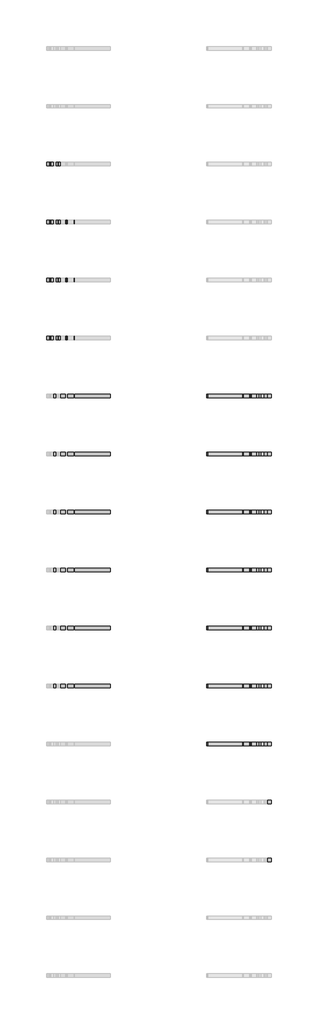
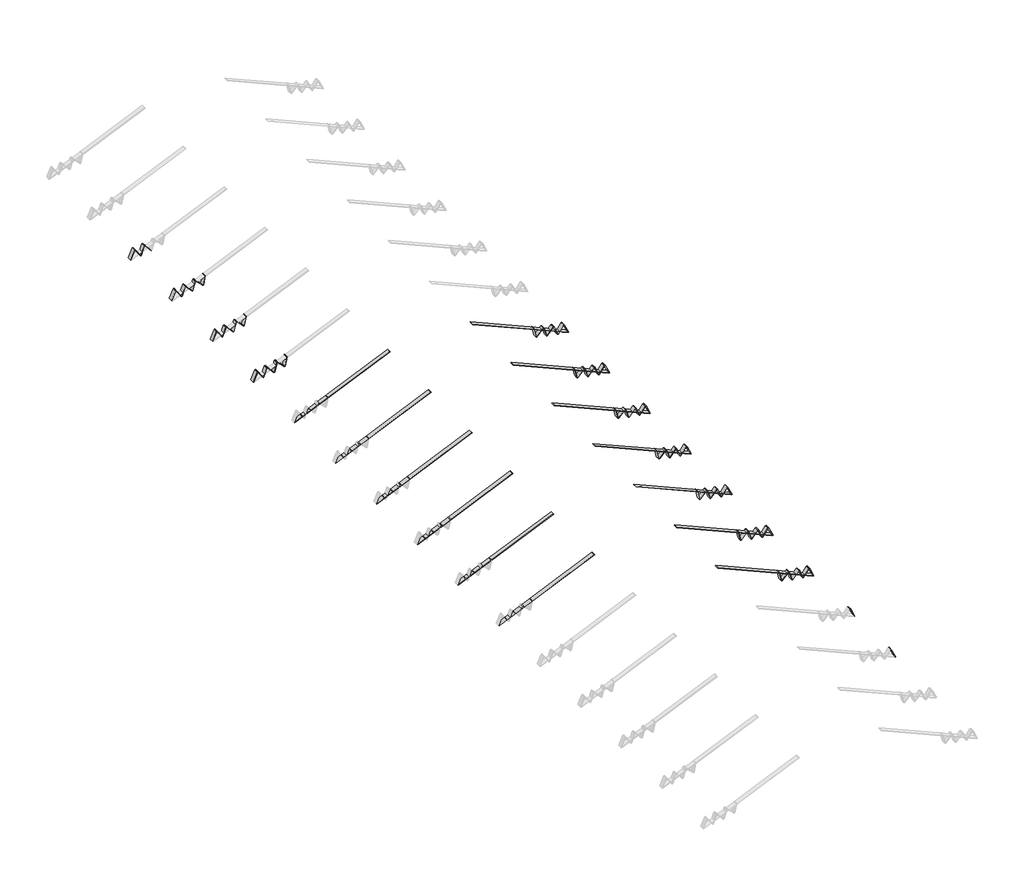
# One storey, part 3 of 4: 89 beams.
"""IFC4 building model written with IfcOpenShell, lengths in millimetres."""

import ifcopenshell
import ifcopenshell.guid

model = None  # the IFC model being written
_history = None  # IfcOwnerHistory: only IFC2X3 demands one
_inside = {}  # id of a spatial element -> (the spatial element, [elements in it])
_under = {}  # id of a project, library or spatial element -> (it, [spatial elements below it])
_declared = {}  # id of a project -> (the project, [libraries it declares])
_typed = {}  # id of a type object -> (the type object, [elements of that type])
_made_of = {}  # id of a material, layer set ... -> (it, [elements and type objects made of it])


def new_model(schema):
    """Start an empty IFC model of exactly this schema.

    Asked for "IFC4X3", IfcOpenShell would pick the latest addendum, in which some entities
    have other attributes; the version numbers below select the first issue.
    IFC2X3 requires an IfcOwnerHistory on every rooted entity: one is made here for all.
    """
    global model, _history
    if schema == "IFC4X3":
        model = ifcopenshell.file(schema_version=(4, 3, 0, 0))
    else:
        model = ifcopenshell.file(schema=schema)
    _inside.clear()
    _under.clear()
    _declared.clear()
    _typed.clear()
    _made_of.clear()
    _history = None
    if model.schema == "IFC2X3":
        org = make("IfcOrganization", Name="unknown")
        user = make(
            "IfcPersonAndOrganization",
            ThePerson=make("IfcPerson", FamilyName="unknown"),
            TheOrganization=org,
        )
        app = make(
            "IfcApplication",
            ApplicationDeveloper=org,
            Version="unknown",
            ApplicationFullName="unknown",
            ApplicationIdentifier="unknown",
        )
        _history = make(
            "IfcOwnerHistory",
            OwningUser=user,
            OwningApplication=app,
            ChangeAction="ADDED",
            CreationDate=0,
        )
    return model


def make(cls, **values):
    """One entity of the class cls with the attributes given. An attribute that is None is left unset."""
    return model.create_entity(
        cls, **{name: value for name, value in values.items() if value is not None}
    )


def rooted(cls, **values):
    """An entity with a GlobalId (a new one), such as an element, a storey or a relation."""
    return make(cls, GlobalId=ifcopenshell.guid.new(), OwnerHistory=_history, **values)


def si_unit(unit_type, name, prefix=None):
    """IfcSIUnit, for example si_unit("LENGTHUNIT", "METRE", prefix="MILLI")."""
    return make("IfcSIUnit", UnitType=unit_type, Prefix=prefix, Name=name)


def assignment(units):
    """IfcUnitAssignment: the units of a project."""
    return None if units is None else make("IfcUnitAssignment", Units=units)


def point(xyz):
    """IfcCartesianPoint."""
    return None if xyz is None else make("IfcCartesianPoint", Coordinates=xyz)


def direction(xyz):
    """IfcDirection."""
    return None if xyz is None else make("IfcDirection", DirectionRatios=xyz)


def frame(location, z_axis=None, x_axis=None):
    """IfcAxis2Placement3D, a coordinate frame: its origin and axes. An axis left out is left unset."""
    return make(
        "IfcAxis2Placement3D",
        Location=point(location),
        Axis=direction(z_axis),
        RefDirection=direction(x_axis),
    )


def frame_2d(location, x_axis=None):
    """IfcAxis2Placement2D, a coordinate frame in the plane: its origin and x axis."""
    return make(
        "IfcAxis2Placement2D", Location=point(location), RefDirection=direction(x_axis)
    )


def origin():
    """The frame at (0, 0, 0) with its axes left unset."""
    return frame((0.0, 0.0, 0.0))


def place(relative_to, where):
    """IfcLocalPlacement: puts the frame where relative to a parent placement (None: the world)."""
    return make(
        "IfcLocalPlacement", PlacementRelTo=relative_to, RelativePlacement=where
    )


def context(
    kind, dimensions, precision=None, world=None, true_north=None, identifier=None
):
    """IfcGeometricRepresentationContext, for example the 3D "Model" context."""
    return make(
        "IfcGeometricRepresentationContext",
        ContextIdentifier=identifier,
        ContextType=kind,
        CoordinateSpaceDimension=dimensions,
        Precision=precision,
        WorldCoordinateSystem=world,
        TrueNorth=true_north,
    )


def project(units=None, contexts=None):
    """IfcProject with its units and contexts."""
    return rooted(
        "IfcProject",
        Name="project",
        RepresentationContexts=contexts,
        UnitsInContext=assignment(units),
    )


def spatial(cls, under=None, at=None, **own):
    """A site, building, storey or space (cls), placed at a placement, below another one or the project."""
    s = rooted(cls, ObjectPlacement=at, **own)
    if under is not None:
        _under.setdefault(under.id(), (under, []))[1].append(s)
    return s


def polyline(points):
    """IfcPolyline through the points."""
    return make("IfcPolyline", Points=[point(p) for p in points])


def circle_curve(where, radius):
    """IfcCircle in the frame where."""
    return make("IfcCircle", Position=where, Radius=radius)


def trimmed(basis, trim1, trim2, sense, master):
    """IfcTrimmedCurve: the piece of a basis curve between two trims."""
    return make(
        "IfcTrimmedCurve",
        BasisCurve=basis,
        Trim1=trim1,
        Trim2=trim2,
        SenseAgreement=sense,
        MasterRepresentation=master,
    )


def segment(curve, same_sense, transition):
    """IfcCompositeCurveSegment."""
    return make(
        "IfcCompositeCurveSegment",
        Transition=transition,
        SameSense=same_sense,
        ParentCurve=curve,
    )


def composite_curve(segments, self_intersect=None):
    """IfcCompositeCurve: segments joined end to end."""
    return make("IfcCompositeCurve", Segments=segments, SelfIntersect=self_intersect)


def outline(outer, holes=None, kind="AREA"):
    """IfcArbitraryClosedProfileDef: a profile drawn as a closed curve; with holes, ...WithVoids."""
    if holes is None:
        return make("IfcArbitraryClosedProfileDef", ProfileType=kind, OuterCurve=outer)
    return make(
        "IfcArbitraryProfileDefWithVoids",
        ProfileType=kind,
        OuterCurve=outer,
        InnerCurves=holes,
    )


def extrude(swept, where, along, depth):
    """IfcExtrudedAreaSolid: the profile swept, set in the frame where, extruded along a direction by depth."""
    return make(
        "IfcExtrudedAreaSolid",
        SweptArea=swept,
        Position=where,
        ExtrudedDirection=direction(along),
        Depth=depth,
    )


def shape(context_of_items, identifier, shape_type, items):
    """IfcShapeRepresentation: the items that make up one representation, for example the "Body"."""
    return make(
        "IfcShapeRepresentation",
        ContextOfItems=context_of_items,
        RepresentationIdentifier=identifier,
        RepresentationType=shape_type,
        Items=items,
    )


def source(mapping_origin, context_of_items, identifier, shape_type, items):
    """IfcRepresentationMap: a shape defined once, which mapped items show again and again."""
    return make(
        "IfcRepresentationMap",
        MappingOrigin=mapping_origin,
        MappedRepresentation=shape(context_of_items, identifier, shape_type, items),
    )


def transform(
    local_origin,
    x_axis=None,
    y_axis=None,
    z_axis=None,
    scale=None,
    scale2=None,
    scale3=None,
    uniform=True,
):
    """IfcCartesianTransformationOperator3D, or its non-uniform kind. x_axis, y_axis, z_axis: its Axis1, 2, 3."""
    if uniform:
        return make(
            "IfcCartesianTransformationOperator3D",
            Axis1=direction(x_axis),
            Axis2=direction(y_axis),
            LocalOrigin=point(local_origin),
            Scale=scale,
            Axis3=direction(z_axis),
        )
    return make(
        "IfcCartesianTransformationOperator3DnonUniform",
        Axis1=direction(x_axis),
        Axis2=direction(y_axis),
        LocalOrigin=point(local_origin),
        Scale=scale,
        Axis3=direction(z_axis),
        Scale2=scale2,
        Scale3=scale3,
    )


def mapped(mapping_source, mapping_target):
    """IfcMappedItem: shows the shape of a source again, moved by a transform."""
    return make(
        "IfcMappedItem", MappingSource=mapping_source, MappingTarget=mapping_target
    )


def made_of(thing, what):
    """Note that an element or type object is made of a material, layer set ...; save() writes the relation."""
    if what is not None:
        _made_of.setdefault(what.id(), (what, []))[1].append(thing)
    return thing


def element(
    cls,
    number,
    at=None,
    inside=None,
    cuts=None,
    type_object=None,
    material=None,
    context=None,
    identifier="Body",
    shape_type=None,
    held_by="IfcProductDefinitionShape",
    body=None,
    shapes=None,
    **own,
):
    """One element of the class cls, such as IfcWall. Its Tag is "e" and its number.

    at: its placement. inside: the storey or other place that contains it. cuts: it is an
    opening in that element (IfcRelVoidsElement). A single representation is given by context,
    identifier, shape_type and body (its items); several are given by shapes. held_by: the class
    of the entity that holds the representations. save() writes the other relations.
    """
    e = rooted(cls, Tag="e%d" % number, ObjectPlacement=at, **own)
    if body is not None:
        shapes = [shape(context, identifier, shape_type, body)]
    if shapes is not None:
        e.Representation = make(held_by, Representations=shapes)
    if inside is not None:
        _inside.setdefault(inside.id(), (inside, []))[1].append(e)
    if cuts is not None:
        rooted(
            "IfcRelVoidsElement", RelatingBuildingElement=cuts, RelatedOpeningElement=e
        )
    if type_object is not None:
        _typed.setdefault(type_object.id(), (type_object, []))[1].append(e)
    return made_of(e, material)


def aggregate(whole, parts):
    """IfcRelAggregates: a whole, such as a stair, and the parts it consists of."""
    return rooted("IfcRelAggregates", RelatingObject=whole, RelatedObjects=parts)


def save(model, path):
    """Write the relations noted so far, then the file.

    IfcRelAggregates (storeys below a building ...), IfcRelContainedInSpatialStructure (elements
    in a storey), IfcRelDefinesByType, IfcRelAssociatesMaterial and IfcRelDeclares: one each for
    every whole, place, type object, material and project.
    """
    for whole, parts in _under.values():
        aggregate(whole, parts)
    for where, things in _inside.values():
        rooted(
            "IfcRelContainedInSpatialStructure",
            RelatedElements=things,
            RelatingStructure=where,
        )
    for kind, things in _typed.values():
        rooted("IfcRelDefinesByType", RelatedObjects=things, RelatingType=kind)
    for what, things in _made_of.values():
        rooted("IfcRelAssociatesMaterial", RelatedObjects=things, RelatingMaterial=what)
    for by, libraries in _declared.values():
        rooted("IfcRelDeclares", RelatingContext=by, RelatedDefinitions=libraries)
    model.write(path)


def placa_diagonal_a71479e9(model_context):
    return source(origin(), model_context, "Body", "SweptSolid", [
        extrude(outline(polyline([(161.178496, 75.0), (161.178496, -75.0), (-185.3041805, -75.0), (-185.3041805, 75.0), (161.178496, 75.0)])), frame((0.0, 0.0, -4.0), z_axis=(0.0, 0.0, 1.0), x_axis=(1.0, 0.0, 0.0)), (0.0, 0.0, 1.0), 8.0),
    ])


def placa_diagonal_67ce8334(model_context):
    return source(origin(), model_context, "Body", "SweptSolid", [
        extrude(outline(polyline([(162.9623469, 75.0), (162.9623469, -75.0), (-162.6761246, -75.0), (-162.6761246, 75.0), (162.9623469, 75.0)])), frame((0.0, 0.0, -4.0), z_axis=(0.0, 0.0, 1.0), x_axis=(1.0, 0.0, 0.0)), (0.0, 0.0, 1.0), 8.0),
    ])


def placa_diagonal_af2a04a3(model_context):
    return source(origin(), model_context, "Body", "SweptSolid", [
        extrude(outline(polyline([(165.1705216, 75.0), (165.1705216, -75.0), (-165.4962729, -75.0), (-165.4962729, 75.0), (165.1705216, 75.0)])), frame((0.0, 0.0, -4.0), z_axis=(0.0, 0.0, 1.0), x_axis=(1.0, 0.0, 0.0)), (0.0, 0.0, 1.0), 8.0),
    ])


def placa_diagonal_fb53ba7d(model_context):
    return source(origin(), model_context, "Body", "SweptSolid", [
        extrude(outline(polyline([(169.971959, 75.0), (169.971959, -75.0), (-169.5739242, -75.0), (-169.5739242, 75.0), (169.971959, 75.0)])), frame((0.0, 0.0, -4.0), z_axis=(0.0, 0.0, 1.0), x_axis=(1.0, 0.0, 0.0)), (0.0, 0.0, 1.0), 8.0),
    ])


def placa_diagonal_d1da0e1c(model_context):
    return source(origin(), model_context, "Body", "SweptSolid", [
        extrude(outline(polyline([(165.1705221, 75.0), (165.1705221, -75.0), (-165.4962734, -75.0), (-165.4962734, 75.0), (165.1705221, 75.0)])), frame((0.0, 0.0, -4.0), z_axis=(0.0, 0.0, 1.0), x_axis=(1.0, 0.0, 0.0)), (0.0, 0.0, 1.0), 8.0),
    ])


def placa_diagonal_6d03bdc5(model_context):
    return source(origin(), model_context, "Body", "SweptSolid", [
        extrude(outline(polyline([(191.209825, 75.0), (191.209825, -75.0), (-166.9394885, -75.0), (-166.9394885, 75.0), (191.209825, 75.0)])), frame((0.0, 0.0, -4.0), z_axis=(0.0, 0.0, 1.0), x_axis=(1.0, 0.0, 0.0)), (0.0, 0.0, 1.0), 8.0),
    ])


def placa_diagonal_30fa4039(model_context):
    return source(origin(), model_context, "Body", "SweptSolid", [
        extrude(outline(polyline([(167.0675386, 75.0), (167.0675386, -75.0), (-167.4240159, -75.0), (-167.4240159, 75.0), (167.0675386, 75.0)])), frame((0.0, 0.0, -4.0), z_axis=(0.0, 0.0, 1.0), x_axis=(1.0, 0.0, 0.0)), (0.0, 0.0, 1.0), 8.0),
    ])


def placa_diagonal_ded414cc(model_context):
    return source(origin(), model_context, "Body", "SweptSolid", [
        extrude(outline(polyline([(167.4240165, 75.0), (167.4240165, -75.0), (-167.0675392, -75.0), (-167.0675392, 75.0), (167.4240165, 75.0)])), frame((0.0, 0.0, -4.0), z_axis=(0.0, 0.0, 1.0), x_axis=(1.0, 0.0, 0.0)), (0.0, 0.0, 1.0), 8.0),
    ])


def placa_diagonal_4690b74a(model_context):
    return source(origin(), model_context, "Body", "SweptSolid", [
        extrude(outline(polyline([(167.0675389, 75.0), (167.0675389, -75.0), (-167.4240162, -75.0), (-167.4240162, 75.0), (167.0675389, 75.0)])), frame((0.0, 0.0, -4.0), z_axis=(0.0, 0.0, 1.0), x_axis=(1.0, 0.0, 0.0)), (0.0, 0.0, 1.0), 8.0),
    ])


def placa_diagonal_aaf0c3b6(model_context):
    return source(origin(), model_context, "Body", "SweptSolid", [
        extrude(outline(polyline([(167.4240163, 75.0), (167.4240163, -75.0), (-167.067539, -75.0), (-167.067539, 75.0), (167.4240163, 75.0)])), frame((0.0, 0.0, -4.0), z_axis=(0.0, 0.0, 1.0), x_axis=(1.0, 0.0, 0.0)), (0.0, 0.0, 1.0), 8.0),
    ])


model = new_model("IFC4")

# Units and contexts
model_context = context("Model", 3, world=origin())
ifc_project = project(units=[si_unit("LENGTHUNIT", "METRE", prefix="MILLI")], contexts=[model_context])

# Site, building, storey
site = spatial("IfcSite", under=ifc_project)
building = spatial("IfcBuilding", under=site)
storey = spatial("IfcBuildingStorey", under=building, Name="Nível 4", Elevation=48165.0)

# Beams
placement = place(None, origin())
element("IfcBeam", 1, ObjectType="Placa : banzo", at=placement, inside=storey, context=model_context, shape_type="SweptSolid", body=[
    extrude(outline(composite_curve([segment(polyline([(48158.5516223, 8114.9704041), (48174.5198715, 8115.9778843)]), True, "CONTINUOUS"), segment(trimmed(circle_curve(frame_2d((53506.1312788, 8452.3636953)), 5342.2126139), [point((48174.5198715, 8115.9778843))], [point((49646.1683419, 4759.1372282))], True, "CARTESIAN"), True, "CONTINUOUS"), segment(polyline([(49646.1683419, 4759.1372282), (49634.6077, 4748.0759643)]), True, "CONTINUOUS"), segment(trimmed(circle_curve(frame_2d((53506.1312788, 8452.3636953)), 5358.2126139), [point((49634.6077, 4748.0759643))], [point((48158.5516223, 8114.9704041))], False, "CARTESIAN"), True, "CONTINUOUS")], self_intersect=False)), frame((0.0, -2178.5623634, 0.0), z_axis=(0.0, 1.0, 0.0), x_axis=(0.0, 0.0, 1.0)), (0.0, 0.0, 1.0), 150.0),
])
element("IfcBeam", 2, ObjectType="Placa : banzo", at=placement, inside=storey, context=model_context, shape_type="SweptSolid", body=[
    extrude(outline(composite_curve([segment(polyline([(49634.6077, 1843.8240278), (49646.1683419, 1832.762764)]), True, "CONTINUOUS"), segment(trimmed(circle_curve(frame_2d((53506.1312788, -1860.4637031)), 5342.2126139), [point((49646.1683419, 1832.762764))], [point((48174.5198715, -1524.0778921))], True, "CARTESIAN"), True, "CONTINUOUS"), segment(polyline([(48174.5198715, -1524.0778921), (48158.5516223, -1523.070412)]), True, "CONTINUOUS"), segment(trimmed(circle_curve(frame_2d((53506.1312788, -1860.4637031)), 5358.2126139), [point((48158.5516223, -1523.070412))], [point((49634.6077, 1843.8240278))], False, "CARTESIAN"), True, "CONTINUOUS")], self_intersect=False)), frame((0.0, -2178.5623634, 0.0), z_axis=(0.0, 1.0, 0.0), x_axis=(0.0, 0.0, 1.0)), (0.0, 0.0, 1.0), 150.0),
])
element("IfcBeam", 3, ObjectType="Placa : banzo", at=placement, inside=storey, context=model_context, shape_type="SweptSolid", body=[
    extrude(outline(composite_curve([segment(polyline([(48158.5516223, 8114.9704041), (48174.5198715, 8115.9778843)]), True, "CONTINUOUS"), segment(trimmed(circle_curve(frame_2d((53506.1312788, 8452.3636953)), 5342.2126139), [point((48174.5198715, 8115.9778843))], [point((49646.1683419, 4759.1372282))], True, "CARTESIAN"), True, "CONTINUOUS"), segment(polyline([(49646.1683419, 4759.1372282), (49634.6077, 4748.0759643)]), True, "CONTINUOUS"), segment(trimmed(circle_curve(frame_2d((53506.1312788, 8452.3636953)), 5358.2126139), [point((49634.6077, 4748.0759643))], [point((48158.5516223, 8114.9704041))], False, "CARTESIAN"), True, "CONTINUOUS")], self_intersect=False)), frame((0.0, -4678.5623634, 0.0), z_axis=(0.0, 1.0, 0.0), x_axis=(0.0, 0.0, 1.0)), (0.0, 0.0, 1.0), 150.0),
])
element("IfcBeam", 4, ObjectType="Placa : banzo", at=placement, inside=storey, context=model_context, shape_type="SweptSolid", body=[
    extrude(outline(composite_curve([segment(polyline([(49634.6077, 1843.8240278), (49646.1683419, 1832.762764)]), True, "CONTINUOUS"), segment(trimmed(circle_curve(frame_2d((53506.1312788, -1860.4637031)), 5342.2126139), [point((49646.1683419, 1832.762764))], [point((48174.5198715, -1524.0778921))], True, "CARTESIAN"), True, "CONTINUOUS"), segment(polyline([(48174.5198715, -1524.0778921), (48158.5516223, -1523.070412)]), True, "CONTINUOUS"), segment(trimmed(circle_curve(frame_2d((53506.1312788, -1860.4637031)), 5358.2126139), [point((48158.5516223, -1523.070412))], [point((49634.6077, 1843.8240278))], False, "CARTESIAN"), True, "CONTINUOUS")], self_intersect=False)), frame((0.0, -4678.5623634, 0.0), z_axis=(0.0, 1.0, 0.0), x_axis=(0.0, 0.0, 1.0)), (0.0, 0.0, 1.0), 150.0),
])
element("IfcBeam", 5, ObjectType="Placa : banzo", at=placement, inside=storey, context=model_context, shape_type="SweptSolid", body=[
    extrude(outline(composite_curve([segment(polyline([(48158.5516223, 8114.9704041), (48174.5198715, 8115.9778843)]), True, "CONTINUOUS"), segment(trimmed(circle_curve(frame_2d((53506.1312788, 8452.3636953)), 5342.2126139), [point((48174.5198715, 8115.9778843))], [point((49646.1683419, 4759.1372282))], True, "CARTESIAN"), True, "CONTINUOUS"), segment(polyline([(49646.1683419, 4759.1372282), (49634.6077, 4748.0759643)]), True, "CONTINUOUS"), segment(trimmed(circle_curve(frame_2d((53506.1312788, 8452.3636953)), 5358.2126139), [point((49634.6077, 4748.0759643))], [point((48158.5516223, 8114.9704041))], False, "CARTESIAN"), True, "CONTINUOUS")], self_intersect=False)), frame((0.0, -7178.5623634, 0.0), z_axis=(0.0, 1.0, 0.0), x_axis=(0.0, 0.0, 1.0)), (0.0, 0.0, 1.0), 150.0),
])
element("IfcBeam", 6, ObjectType="Placa : banzo", at=placement, inside=storey, context=model_context, shape_type="SweptSolid", body=[
    extrude(outline(composite_curve([segment(polyline([(49634.6077, 1843.8240278), (49646.1683419, 1832.762764)]), True, "CONTINUOUS"), segment(trimmed(circle_curve(frame_2d((53506.1312788, -1860.4637031)), 5342.2126139), [point((49646.1683419, 1832.762764))], [point((48174.5198715, -1524.0778921))], True, "CARTESIAN"), True, "CONTINUOUS"), segment(polyline([(48174.5198715, -1524.0778921), (48158.5516223, -1523.070412)]), True, "CONTINUOUS"), segment(trimmed(circle_curve(frame_2d((53506.1312788, -1860.4637031)), 5358.2126139), [point((48158.5516223, -1523.070412))], [point((49634.6077, 1843.8240278))], False, "CARTESIAN"), True, "CONTINUOUS")], self_intersect=False)), frame((0.0, -7178.5623634, 0.0), z_axis=(0.0, 1.0, 0.0), x_axis=(0.0, 0.0, 1.0)), (0.0, 0.0, 1.0), 150.0),
])
element("IfcBeam", 7, ObjectType="Placa : banzo", at=placement, inside=storey, context=model_context, shape_type="SweptSolid", body=[
    extrude(outline(composite_curve([segment(polyline([(48158.5516223, 8114.9704041), (48174.5198715, 8115.9778843)]), True, "CONTINUOUS"), segment(trimmed(circle_curve(frame_2d((53506.1312788, 8452.3636953)), 5342.2126139), [point((48174.5198715, 8115.9778843))], [point((49646.1683419, 4759.1372282))], True, "CARTESIAN"), True, "CONTINUOUS"), segment(polyline([(49646.1683419, 4759.1372282), (49634.6077, 4748.0759643)]), True, "CONTINUOUS"), segment(trimmed(circle_curve(frame_2d((53506.1312788, 8452.3636953)), 5358.2126139), [point((49634.6077, 4748.0759643))], [point((48158.5516223, 8114.9704041))], False, "CARTESIAN"), True, "CONTINUOUS")], self_intersect=False)), frame((0.0, -9678.5623634, 0.0), z_axis=(0.0, 1.0, 0.0), x_axis=(0.0, 0.0, 1.0)), (0.0, 0.0, 1.0), 150.0),
])
element("IfcBeam", 8, ObjectType="Placa : banzo", at=placement, inside=storey, context=model_context, shape_type="SweptSolid", body=[
    extrude(outline(composite_curve([segment(polyline([(49634.6077, 1843.8240278), (49646.1683419, 1832.762764)]), True, "CONTINUOUS"), segment(trimmed(circle_curve(frame_2d((53506.1312788, -1860.4637031)), 5342.2126139), [point((49646.1683419, 1832.762764))], [point((48174.5198715, -1524.0778921))], True, "CARTESIAN"), True, "CONTINUOUS"), segment(polyline([(48174.5198715, -1524.0778921), (48158.5516223, -1523.070412)]), True, "CONTINUOUS"), segment(trimmed(circle_curve(frame_2d((53506.1312788, -1860.4637031)), 5358.2126139), [point((48158.5516223, -1523.070412))], [point((49634.6077, 1843.8240278))], False, "CARTESIAN"), True, "CONTINUOUS")], self_intersect=False)), frame((0.0, -9678.5623634, 0.0), z_axis=(0.0, 1.0, 0.0), x_axis=(0.0, 0.0, 1.0)), (0.0, 0.0, 1.0), 150.0),
])
element("IfcBeam", 9, ObjectType="Placa : banzo", at=placement, inside=storey, context=model_context, shape_type="SweptSolid", body=[
    extrude(outline(composite_curve([segment(polyline([(48158.5516223, 8114.9704041), (48174.5198715, 8115.9778843)]), True, "CONTINUOUS"), segment(trimmed(circle_curve(frame_2d((53506.1312788, 8452.3636953)), 5342.2126139), [point((48174.5198715, 8115.9778843))], [point((49646.1683419, 4759.1372282))], True, "CARTESIAN"), True, "CONTINUOUS"), segment(polyline([(49646.1683419, 4759.1372282), (49634.6077, 4748.0759643)]), True, "CONTINUOUS"), segment(trimmed(circle_curve(frame_2d((53506.1312788, 8452.3636953)), 5358.2126139), [point((49634.6077, 4748.0759643))], [point((48158.5516223, 8114.9704041))], False, "CARTESIAN"), True, "CONTINUOUS")], self_intersect=False)), frame((0.0, -12178.5623634, 0.0), z_axis=(0.0, 1.0, 0.0), x_axis=(0.0, 0.0, 1.0)), (0.0, 0.0, 1.0), 150.0),
])
element("IfcBeam", 10, ObjectType="Placa : banzo", at=placement, inside=storey, context=model_context, shape_type="SweptSolid", body=[
    extrude(outline(composite_curve([segment(polyline([(49634.6077, 1843.8240278), (49646.1683419, 1832.762764)]), True, "CONTINUOUS"), segment(trimmed(circle_curve(frame_2d((53506.1312788, -1860.4637031)), 5342.2126139), [point((49646.1683419, 1832.762764))], [point((48174.5198715, -1524.0778921))], True, "CARTESIAN"), True, "CONTINUOUS"), segment(polyline([(48174.5198715, -1524.0778921), (48158.5516223, -1523.070412)]), True, "CONTINUOUS"), segment(trimmed(circle_curve(frame_2d((53506.1312788, -1860.4637031)), 5358.2126139), [point((48158.5516223, -1523.070412))], [point((49634.6077, 1843.8240278))], False, "CARTESIAN"), True, "CONTINUOUS")], self_intersect=False)), frame((0.0, -12178.5623634, 0.0), z_axis=(0.0, 1.0, 0.0), x_axis=(0.0, 0.0, 1.0)), (0.0, 0.0, 1.0), 150.0),
])
element("IfcBeam", 11, ObjectType="Placa : banzo", at=placement, inside=storey, context=model_context, shape_type="SweptSolid", body=[
    extrude(outline(composite_curve([segment(polyline([(48158.5516223, 8114.9704041), (48174.5198715, 8115.9778843)]), True, "CONTINUOUS"), segment(trimmed(circle_curve(frame_2d((53506.1312788, 8452.3636953)), 5342.2126139), [point((48174.5198715, 8115.9778843))], [point((49646.1683419, 4759.1372282))], True, "CARTESIAN"), True, "CONTINUOUS"), segment(polyline([(49646.1683419, 4759.1372282), (49634.6077, 4748.0759643)]), True, "CONTINUOUS"), segment(trimmed(circle_curve(frame_2d((53506.1312788, 8452.3636953)), 5358.2126139), [point((49634.6077, 4748.0759643))], [point((48158.5516223, 8114.9704041))], False, "CARTESIAN"), True, "CONTINUOUS")], self_intersect=False)), frame((0.0, -14678.5623634, 0.0), z_axis=(0.0, 1.0, 0.0), x_axis=(0.0, 0.0, 1.0)), (0.0, 0.0, 1.0), 150.0),
])
element("IfcBeam", 12, ObjectType="Placa : banzo", at=placement, inside=storey, context=model_context, shape_type="SweptSolid", body=[
    extrude(outline(composite_curve([segment(polyline([(49634.6077, 1843.8240278), (49646.1683419, 1832.762764)]), True, "CONTINUOUS"), segment(trimmed(circle_curve(frame_2d((53506.1312788, -1860.4637031)), 5342.2126139), [point((49646.1683419, 1832.762764))], [point((48174.5198715, -1524.0778921))], True, "CARTESIAN"), True, "CONTINUOUS"), segment(polyline([(48174.5198715, -1524.0778921), (48158.5516223, -1523.070412)]), True, "CONTINUOUS"), segment(trimmed(circle_curve(frame_2d((53506.1312788, -1860.4637031)), 5358.2126139), [point((48158.5516223, -1523.070412))], [point((49634.6077, 1843.8240278))], False, "CARTESIAN"), True, "CONTINUOUS")], self_intersect=False)), frame((0.0, -14678.5623634, 0.0), z_axis=(0.0, 1.0, 0.0), x_axis=(0.0, 0.0, 1.0)), (0.0, 0.0, 1.0), 150.0),
])
element("IfcBeam", 13, ObjectType="Placa : banzo", at=placement, inside=storey, context=model_context, shape_type="SweptSolid", body=[
    extrude(outline(composite_curve([segment(polyline([(48158.5516223, 8114.9704041), (48174.5198715, 8115.9778843)]), True, "CONTINUOUS"), segment(trimmed(circle_curve(frame_2d((53506.1312788, 8452.3636953)), 5342.2126139), [point((48174.5198715, 8115.9778843))], [point((49646.1683419, 4759.1372282))], True, "CARTESIAN"), True, "CONTINUOUS"), segment(polyline([(49646.1683419, 4759.1372282), (49634.6077, 4748.0759643)]), True, "CONTINUOUS"), segment(trimmed(circle_curve(frame_2d((53506.1312788, 8452.3636953)), 5358.2126139), [point((49634.6077, 4748.0759643))], [point((48158.5516223, 8114.9704041))], False, "CARTESIAN"), True, "CONTINUOUS")], self_intersect=False)), frame((0.0, -17178.5623634, 0.0), z_axis=(0.0, 1.0, 0.0), x_axis=(0.0, 0.0, 1.0)), (0.0, 0.0, 1.0), 150.0),
])
placa_diagonal_shape = placa_diagonal_a71479e9(model_context)
element("IfcBeam", 14, ObjectType="Placa : diagonal", at=placement, inside=storey, context=model_context, shape_type="MappedRepresentation", body=[
    mapped(placa_diagonal_shape, transform((-1468.5029422, 7896.4376366, 48342.5238752), x_axis=(0.4074605623535313, 0.0, 0.9132228042085588), y_axis=(0.0, -1.0, 0.0), z_axis=(0.9132228042085588, 0.0, -0.4074605623535313))),
])
element("IfcBeam", 15, ObjectType="Placa : diagonal", at=placement, inside=storey, context=model_context, shape_type="MappedRepresentation", body=[
    mapped(placa_diagonal_shape, transform((-1468.5029422, 5396.4376366, 48342.5238752), x_axis=(0.4074605623535313, 0.0, 0.9132228042085588), y_axis=(0.0, -1.0, 0.0), z_axis=(0.9132228042085588, 0.0, -0.4074605623535313))),
])
element("IfcBeam", 16, ObjectType="Placa : diagonal", at=placement, inside=storey, context=model_context, shape_type="MappedRepresentation", body=[
    mapped(placa_diagonal_shape, transform((-1468.5029422, 2896.4376366, 48342.5238752), x_axis=(0.4074605623535313, 0.0, 0.9132228042085588), y_axis=(0.0, -1.0, 0.0), z_axis=(0.9132228042085588, 0.0, -0.4074605623535313))),
])
element("IfcBeam", 17, ObjectType="Placa : diagonal", at=placement, inside=storey, context=model_context, shape_type="MappedRepresentation", body=[
    mapped(placa_diagonal_shape, transform((-1468.5029422, 396.4376366, 48342.5238752), x_axis=(0.4074605623535313, 0.0, 0.9132228042085588), y_axis=(0.0, -1.0, 0.0), z_axis=(0.9132228042085588, 0.0, -0.4074605623535313))),
])
placa_diagonal_2_shape = placa_diagonal_67ce8334(model_context)
element("IfcBeam", 18, ObjectType="Placa : diagonal", at=placement, inside=storey, context=model_context, shape_type="MappedRepresentation", body=[
    mapped(placa_diagonal_2_shape, transform((-1292.3410904, 7896.4376366, 48354.815057), x_axis=(0.5398932132172984, 0.0, -0.8417335197803998), y_axis=(0.0, -1.0, 0.0), z_axis=(-0.8417335197803998, 0.0, -0.5398932132172984))),
])
element("IfcBeam", 19, ObjectType="Placa : diagonal", at=placement, inside=storey, context=model_context, shape_type="MappedRepresentation", body=[
    mapped(placa_diagonal_2_shape, transform((-1292.3410904, 5396.4376366, 48354.815057), x_axis=(0.5398932132172984, 0.0, -0.8417335197803998), y_axis=(0.0, -1.0, 0.0), z_axis=(-0.8417335197803998, 0.0, -0.5398932132172984))),
])
element("IfcBeam", 20, ObjectType="Placa : diagonal", at=placement, inside=storey, context=model_context, shape_type="MappedRepresentation", body=[
    mapped(placa_diagonal_2_shape, transform((-1292.3410904, 2896.4376366, 48354.815057), x_axis=(0.5398932132172984, 0.0, -0.8417335197803998), y_axis=(0.0, -1.0, 0.0), z_axis=(-0.8417335197803998, 0.0, -0.5398932132172984))),
])
element("IfcBeam", 21, ObjectType="Placa : diagonal", at=placement, inside=storey, context=model_context, shape_type="MappedRepresentation", body=[
    mapped(placa_diagonal_2_shape, transform((-1292.3410904, 396.4376366, 48354.815057), x_axis=(0.5398932132172984, 0.0, -0.8417335197803998), y_axis=(0.0, -1.0, 0.0), z_axis=(-0.8417335197803998, 0.0, -0.5398932132172984))),
])
placa_diagonal_3_shape = placa_diagonal_af2a04a3(model_context)
element("IfcBeam", 22, ObjectType="Placa : diagonal", at=placement, inside=storey, context=model_context, shape_type="MappedRepresentation", body=[
    mapped(placa_diagonal_3_shape, transform((-1127.2550828, 7896.4376366, 48375.8118772), x_axis=(0.3404667803509138, 0.0, 0.940256545564817), y_axis=(0.0, -1.0, 0.0), z_axis=(0.940256545564817, 0.0, -0.3404667803509138))),
])
element("IfcBeam", 23, ObjectType="Placa : diagonal", at=placement, inside=storey, context=model_context, shape_type="MappedRepresentation", body=[
    mapped(placa_diagonal_3_shape, transform((-1127.2550828, 5396.4376366, 48375.8118772), x_axis=(0.3404667803509138, 0.0, 0.940256545564817), y_axis=(0.0, -1.0, 0.0), z_axis=(0.940256545564817, 0.0, -0.3404667803509138))),
])
element("IfcBeam", 24, ObjectType="Placa : diagonal", at=placement, inside=storey, context=model_context, shape_type="MappedRepresentation", body=[
    mapped(placa_diagonal_3_shape, transform((-392.7303205, 5396.4376366, 48535.8666224), x_axis=(0.20085127706480188, 0.0, 0.9796217456250337), y_axis=(0.0, -1.0, 0.0), z_axis=(0.9796217456250337, 0.0, -0.20085127706480188))),
])
element("IfcBeam", 25, ObjectType="Placa : diagonal", at=placement, inside=storey, context=model_context, shape_type="MappedRepresentation", body=[
    mapped(placa_diagonal_3_shape, transform((-1127.2550828, 2896.4376366, 48375.8118772), x_axis=(0.3404667803509138, 0.0, 0.940256545564817), y_axis=(0.0, -1.0, 0.0), z_axis=(0.940256545564817, 0.0, -0.3404667803509138))),
])
element("IfcBeam", 26, ObjectType="Placa : diagonal", at=placement, inside=storey, context=model_context, shape_type="MappedRepresentation", body=[
    mapped(placa_diagonal_3_shape, transform((-392.7303205, 2896.4376366, 48535.8666224), x_axis=(0.20085127706480188, 0.0, 0.9796217456250337), y_axis=(0.0, -1.0, 0.0), z_axis=(0.9796217456250337, 0.0, -0.20085127706480188))),
])
element("IfcBeam", 27, ObjectType="Placa : diagonal", at=placement, inside=storey, context=model_context, shape_type="MappedRepresentation", body=[
    mapped(placa_diagonal_3_shape, transform((-1127.2550828, 396.4376366, 48375.8118772), x_axis=(0.3404667803509138, 0.0, 0.940256545564817), y_axis=(0.0, -1.0, 0.0), z_axis=(0.940256545564817, 0.0, -0.3404667803509138))),
])
element("IfcBeam", 28, ObjectType="Placa : diagonal", at=placement, inside=storey, context=model_context, shape_type="MappedRepresentation", body=[
    mapped(placa_diagonal_3_shape, transform((-392.7303205, 396.4376366, 48535.8666224), x_axis=(0.20085127706480188, 0.0, 0.9796217456250337), y_axis=(0.0, -1.0, 0.0), z_axis=(0.9796217456250337, 0.0, -0.20085127706480188))),
])
placa_diagonal_4_shape = placa_diagonal_fb53ba7d(model_context)
element("IfcBeam", 29, ObjectType="Placa : diagonal", at=placement, inside=storey, context=model_context, shape_type="MappedRepresentation", body=[
    mapped(placa_diagonal_4_shape, transform((-935.6334765, 7896.4376366, 48407.0552778), x_axis=(0.6551223780870831, 0.0, -0.7555227790937377), y_axis=(0.0, -1.0, 0.0), z_axis=(-0.7555227790937377, 0.0, -0.6551223780870831))),
])
element("IfcBeam", 30, ObjectType="Placa : diagonal", at=placement, inside=storey, context=model_context, shape_type="MappedRepresentation", body=[
    mapped(placa_diagonal_4_shape, transform((-935.6334765, 5396.4376366, 48407.0552778), x_axis=(0.6551223780870831, 0.0, -0.7555227790937377), y_axis=(0.0, -1.0, 0.0), z_axis=(-0.7555227790937377, 0.0, -0.6551223780870831))),
])
element("IfcBeam", 31, ObjectType="Placa : diagonal", at=placement, inside=storey, context=model_context, shape_type="MappedRepresentation", body=[
    mapped(placa_diagonal_4_shape, transform((-568.2358431, 5396.4376366, 48487.5623421), x_axis=(0.7081946416059488, 0.0, -0.706017244549042), y_axis=(0.0, -1.0, 0.0), z_axis=(-0.706017244549042, 0.0, -0.7081946416059488))),
])
element("IfcBeam", 32, ObjectType="Placa : diagonal", at=placement, inside=storey, context=model_context, shape_type="MappedRepresentation", body=[
    mapped(placa_diagonal_4_shape, transform((-935.6334765, 2896.4376366, 48407.0552778), x_axis=(0.6551223780870831, 0.0, -0.7555227790937377), y_axis=(0.0, -1.0, 0.0), z_axis=(-0.7555227790937377, 0.0, -0.6551223780870831))),
])
element("IfcBeam", 33, ObjectType="Placa : diagonal", at=placement, inside=storey, context=model_context, shape_type="MappedRepresentation", body=[
    mapped(placa_diagonal_4_shape, transform((-568.2358431, 2896.4376366, 48487.5623421), x_axis=(0.7081946416059488, 0.0, -0.706017244549042), y_axis=(0.0, -1.0, 0.0), z_axis=(-0.706017244549042, 0.0, -0.7081946416059488))),
])
element("IfcBeam", 34, ObjectType="Placa : diagonal", at=placement, inside=storey, context=model_context, shape_type="MappedRepresentation", body=[
    mapped(placa_diagonal_4_shape, transform((-935.6334765, 396.4376366, 48407.0552778), x_axis=(0.6551223780870831, 0.0, -0.7555227790937377), y_axis=(0.0, -1.0, 0.0), z_axis=(-0.7555227790937377, 0.0, -0.6551223780870831))),
])
element("IfcBeam", 35, ObjectType="Placa : diagonal", at=placement, inside=storey, context=model_context, shape_type="MappedRepresentation", body=[
    mapped(placa_diagonal_4_shape, transform((-568.2358431, 396.4376366, 48487.5623421), x_axis=(0.7081946416059488, 0.0, -0.706017244549042), y_axis=(0.0, -1.0, 0.0), z_axis=(-0.706017244549042, 0.0, -0.7081946416059488))),
])
placa_diagonal_5_shape = placa_diagonal_d1da0e1c(model_context)
element("IfcBeam", 36, ObjectType="Placa : diagonal", at=placement, inside=storey, context=model_context, shape_type="MappedRepresentation", body=[
    mapped(placa_diagonal_5_shape, transform((-757.0867023, 5396.4376366, 48442.5030113), x_axis=(0.2713737594345945, 0.0, 0.9624740426059993), y_axis=(0.0, -1.0, 0.0), z_axis=(0.9624740426059993, 0.0, -0.2713737594345945))),
])
element("IfcBeam", 37, ObjectType="Placa : diagonal", at=placement, inside=storey, context=model_context, shape_type="MappedRepresentation", body=[
    mapped(placa_diagonal_5_shape, transform((-757.0867023, 2896.4376366, 48442.5030113), x_axis=(0.2713737594345945, 0.0, 0.9624740426059993), y_axis=(0.0, -1.0, 0.0), z_axis=(0.9624740426059993, 0.0, -0.2713737594345945))),
])
element("IfcBeam", 38, ObjectType="Placa : diagonal", at=placement, inside=storey, context=model_context, shape_type="MappedRepresentation", body=[
    mapped(placa_diagonal_5_shape, transform((-757.0867023, 396.4376366, 48442.5030113), x_axis=(0.2713737594345945, 0.0, 0.9624740426059993), y_axis=(0.0, -1.0, 0.0), z_axis=(0.9624740426059993, 0.0, -0.2713737594345945))),
])
placa_diagonal_6_shape = placa_diagonal_6d03bdc5(model_context)
element("IfcBeam", 39, ObjectType="Placa : diagonal", at=placement, inside=storey, context=model_context, shape_type="MappedRepresentation", body=[
    mapped(placa_diagonal_6_shape, transform((8059.7198757, -2103.5623634, 48338.6280973), x_axis=(0.4189773842608123, 0.0, -0.9079966693099526), y_axis=(0.0, -1.0, 0.0), z_axis=(-0.9079966693099526, 0.0, -0.4189773842608123))),
])
element("IfcBeam", 40, ObjectType="Placa : diagonal", at=placement, inside=storey, context=model_context, shape_type="MappedRepresentation", body=[
    mapped(placa_diagonal_6_shape, transform((8059.7198757, -4603.5623634, 48338.6280973), x_axis=(0.4189773842608123, 0.0, -0.9079966693099526), y_axis=(0.0, -1.0, 0.0), z_axis=(-0.9079966693099526, 0.0, -0.4189773842608123))),
])
element("IfcBeam", 41, ObjectType="Placa : diagonal", at=placement, inside=storey, context=model_context, shape_type="MappedRepresentation", body=[
    mapped(placa_diagonal_6_shape, transform((8059.7198757, -7103.5623634, 48338.6280973), x_axis=(0.4189773842608123, 0.0, -0.9079966693099526), y_axis=(0.0, -1.0, 0.0), z_axis=(-0.9079966693099526, 0.0, -0.4189773842608123))),
])
element("IfcBeam", 42, ObjectType="Placa : diagonal", at=placement, inside=storey, context=model_context, shape_type="MappedRepresentation", body=[
    mapped(placa_diagonal_6_shape, transform((8059.7198757, -9603.5623634, 48338.6280973), x_axis=(0.4189773842608123, 0.0, -0.9079966693099526), y_axis=(0.0, -1.0, 0.0), z_axis=(-0.9079966693099526, 0.0, -0.4189773842608123))),
])
element("IfcBeam", 43, ObjectType="Placa : diagonal", at=placement, inside=storey, context=model_context, shape_type="MappedRepresentation", body=[
    mapped(placa_diagonal_6_shape, transform((8059.7198757, -12103.5623634, 48338.6280973), x_axis=(0.4189773842608123, 0.0, -0.9079966693099526), y_axis=(0.0, -1.0, 0.0), z_axis=(-0.9079966693099526, 0.0, -0.4189773842608123))),
])
element("IfcBeam", 44, ObjectType="Placa : diagonal", at=placement, inside=storey, context=model_context, shape_type="MappedRepresentation", body=[
    mapped(placa_diagonal_6_shape, transform((8059.7198757, -14603.5623634, 48338.6280973), x_axis=(0.4189773842608123, 0.0, -0.9079966693099526), y_axis=(0.0, -1.0, 0.0), z_axis=(-0.9079966693099526, 0.0, -0.4189773842608123))),
])
element("IfcBeam", 45, ObjectType="Placa : diagonal", at=placement, inside=storey, context=model_context, shape_type="MappedRepresentation", body=[
    mapped(placa_diagonal_6_shape, transform((8059.7198757, -17103.5623634, 48338.6280973), x_axis=(0.4189773842608123, 0.0, -0.9079966693099526), y_axis=(0.0, -1.0, 0.0), z_axis=(-0.9079966693099526, 0.0, -0.4189773842608123))),
])
element("IfcBeam", 46, ObjectType="Placa : diagonal", at=placement, inside=storey, context=model_context, shape_type="MappedRepresentation", body=[
    mapped(placa_diagonal_6_shape, transform((8059.7198757, -19603.5623634, 48338.6280973), x_axis=(0.4189773842608123, 0.0, -0.9079966693099526), y_axis=(0.0, -1.0, 0.0), z_axis=(-0.9079966693099526, 0.0, -0.4189773842608123))),
])
element("IfcBeam", 47, ObjectType="Placa : diagonal", at=placement, inside=storey, context=model_context, shape_type="MappedRepresentation", body=[
    mapped(placa_diagonal_6_shape, transform((8059.7198757, -22103.5623634, 48338.6280973), x_axis=(0.4189773842608123, 0.0, -0.9079966693099526), y_axis=(0.0, -1.0, 0.0), z_axis=(-0.9079966693099526, 0.0, -0.4189773842608123))),
])
placa_diagonal_7_shape = placa_diagonal_30fa4039(model_context)
element("IfcBeam", 48, ObjectType="Placa : diagonal", at=placement, inside=storey, context=model_context, shape_type="MappedRepresentation", body=[
    mapped(placa_diagonal_7_shape, transform((7867.9931921, -2103.5623634, 48356.8132581), x_axis=(0.5832804616623758, 0.0, 0.8122708310920229), y_axis=(0.0, -1.0, 0.0), z_axis=(0.8122708310920229, 0.0, -0.5832804616623758))),
])
element("IfcBeam", 49, ObjectType="Placa : diagonal", at=placement, inside=storey, context=model_context, shape_type="MappedRepresentation", body=[
    mapped(placa_diagonal_7_shape, transform((7867.9931921, -4603.5623634, 48356.8132581), x_axis=(0.5832804616623758, 0.0, 0.8122708310920229), y_axis=(0.0, -1.0, 0.0), z_axis=(0.8122708310920229, 0.0, -0.5832804616623758))),
])
element("IfcBeam", 50, ObjectType="Placa : diagonal", at=placement, inside=storey, context=model_context, shape_type="MappedRepresentation", body=[
    mapped(placa_diagonal_7_shape, transform((7867.9931921, -7103.5623634, 48356.8132581), x_axis=(0.5832804616623758, 0.0, 0.8122708310920229), y_axis=(0.0, -1.0, 0.0), z_axis=(0.8122708310920229, 0.0, -0.5832804616623758))),
])
element("IfcBeam", 51, ObjectType="Placa : diagonal", at=placement, inside=storey, context=model_context, shape_type="MappedRepresentation", body=[
    mapped(placa_diagonal_7_shape, transform((7867.9931921, -9603.5623634, 48356.8132581), x_axis=(0.5832804616623758, 0.0, 0.8122708310920229), y_axis=(0.0, -1.0, 0.0), z_axis=(0.8122708310920229, 0.0, -0.5832804616623758))),
])
element("IfcBeam", 52, ObjectType="Placa : diagonal", at=placement, inside=storey, context=model_context, shape_type="MappedRepresentation", body=[
    mapped(placa_diagonal_7_shape, transform((7867.9931921, -12103.5623634, 48356.8132581), x_axis=(0.5832804616623758, 0.0, 0.8122708310920229), y_axis=(0.0, -1.0, 0.0), z_axis=(0.8122708310920229, 0.0, -0.5832804616623758))),
])
element("IfcBeam", 53, ObjectType="Placa : diagonal", at=placement, inside=storey, context=model_context, shape_type="MappedRepresentation", body=[
    mapped(placa_diagonal_7_shape, transform((7867.9931921, -14603.5623634, 48356.8132581), x_axis=(0.5832804616623758, 0.0, 0.8122708310920229), y_axis=(0.0, -1.0, 0.0), z_axis=(0.8122708310920229, 0.0, -0.5832804616623758))),
])
element("IfcBeam", 54, ObjectType="Placa : diagonal", at=placement, inside=storey, context=model_context, shape_type="MappedRepresentation", body=[
    mapped(placa_diagonal_7_shape, transform((7867.9931921, -17103.5623634, 48356.8132581), x_axis=(0.5832804616623758, 0.0, 0.8122708310920229), y_axis=(0.0, -1.0, 0.0), z_axis=(0.8122708310920229, 0.0, -0.5832804616623758))),
])
placa_diagonal_8_shape = placa_diagonal_ded414cc(model_context)
element("IfcBeam", 55, ObjectType="Placa : diagonal", at=placement, inside=storey, context=model_context, shape_type="MappedRepresentation", body=[
    mapped(placa_diagonal_8_shape, transform((7688.6379629, -2103.5623634, 48380.344708), x_axis=(0.3540062158971715, 0.0, -0.935243069531213), y_axis=(0.0, -1.0, 0.0), z_axis=(-0.935243069531213, 0.0, -0.3540062158971715))),
])
element("IfcBeam", 56, ObjectType="Placa : diagonal", at=placement, inside=storey, context=model_context, shape_type="MappedRepresentation", body=[
    mapped(placa_diagonal_8_shape, transform((7321.1773395, -2103.5623634, 48448.7226144), x_axis=(0.2856767726847757, 0.0, -0.9583260309249723), y_axis=(0.0, -1.0, 0.0), z_axis=(-0.9583260309249723, 0.0, -0.2856767726847757))),
])
element("IfcBeam", 57, ObjectType="Placa : diagonal", at=placement, inside=storey, context=model_context, shape_type="MappedRepresentation", body=[
    mapped(placa_diagonal_8_shape, transform((7688.6379629, -4603.5623634, 48380.344708), x_axis=(0.3540062158971715, 0.0, -0.935243069531213), y_axis=(0.0, -1.0, 0.0), z_axis=(-0.935243069531213, 0.0, -0.3540062158971715))),
])
element("IfcBeam", 58, ObjectType="Placa : diagonal", at=placement, inside=storey, context=model_context, shape_type="MappedRepresentation", body=[
    mapped(placa_diagonal_8_shape, transform((7321.1773395, -4603.5623634, 48448.7226144), x_axis=(0.2856767726847757, 0.0, -0.9583260309249723), y_axis=(0.0, -1.0, 0.0), z_axis=(-0.9583260309249723, 0.0, -0.2856767726847757))),
])
element("IfcBeam", 59, ObjectType="Placa : diagonal", at=placement, inside=storey, context=model_context, shape_type="MappedRepresentation", body=[
    mapped(placa_diagonal_8_shape, transform((7688.6379629, -7103.5623634, 48380.344708), x_axis=(0.3540062158971715, 0.0, -0.935243069531213), y_axis=(0.0, -1.0, 0.0), z_axis=(-0.935243069531213, 0.0, -0.3540062158971715))),
])
element("IfcBeam", 60, ObjectType="Placa : diagonal", at=placement, inside=storey, context=model_context, shape_type="MappedRepresentation", body=[
    mapped(placa_diagonal_8_shape, transform((7321.1773395, -7103.5623634, 48448.7226144), x_axis=(0.2856767726847757, 0.0, -0.9583260309249723), y_axis=(0.0, -1.0, 0.0), z_axis=(-0.9583260309249723, 0.0, -0.2856767726847757))),
])
element("IfcBeam", 61, ObjectType="Placa : diagonal", at=placement, inside=storey, context=model_context, shape_type="MappedRepresentation", body=[
    mapped(placa_diagonal_8_shape, transform((7688.6379629, -9603.5623634, 48380.344708), x_axis=(0.3540062158971715, 0.0, -0.935243069531213), y_axis=(0.0, -1.0, 0.0), z_axis=(-0.935243069531213, 0.0, -0.3540062158971715))),
])
element("IfcBeam", 62, ObjectType="Placa : diagonal", at=placement, inside=storey, context=model_context, shape_type="MappedRepresentation", body=[
    mapped(placa_diagonal_8_shape, transform((7321.1773395, -9603.5623634, 48448.7226144), x_axis=(0.2856767726847757, 0.0, -0.9583260309249723), y_axis=(0.0, -1.0, 0.0), z_axis=(-0.9583260309249723, 0.0, -0.2856767726847757))),
])
element("IfcBeam", 63, ObjectType="Placa : diagonal", at=placement, inside=storey, context=model_context, shape_type="MappedRepresentation", body=[
    mapped(placa_diagonal_8_shape, transform((7688.6379629, -12103.5623634, 48380.344708), x_axis=(0.3540062158971715, 0.0, -0.935243069531213), y_axis=(0.0, -1.0, 0.0), z_axis=(-0.935243069531213, 0.0, -0.3540062158971715))),
])
element("IfcBeam", 64, ObjectType="Placa : diagonal", at=placement, inside=storey, context=model_context, shape_type="MappedRepresentation", body=[
    mapped(placa_diagonal_8_shape, transform((7321.1773395, -12103.5623634, 48448.7226144), x_axis=(0.2856767726847757, 0.0, -0.9583260309249723), y_axis=(0.0, -1.0, 0.0), z_axis=(-0.9583260309249723, 0.0, -0.2856767726847757))),
])
element("IfcBeam", 65, ObjectType="Placa : diagonal", at=placement, inside=storey, context=model_context, shape_type="MappedRepresentation", body=[
    mapped(placa_diagonal_8_shape, transform((7688.6379629, -14603.5623634, 48380.344708), x_axis=(0.3540062158971715, 0.0, -0.935243069531213), y_axis=(0.0, -1.0, 0.0), z_axis=(-0.935243069531213, 0.0, -0.3540062158971715))),
])
element("IfcBeam", 66, ObjectType="Placa : diagonal", at=placement, inside=storey, context=model_context, shape_type="MappedRepresentation", body=[
    mapped(placa_diagonal_8_shape, transform((7321.1773395, -14603.5623634, 48448.7226144), x_axis=(0.2856767726847757, 0.0, -0.9583260309249723), y_axis=(0.0, -1.0, 0.0), z_axis=(-0.9583260309249723, 0.0, -0.2856767726847757))),
])
element("IfcBeam", 67, ObjectType="Placa : diagonal", at=placement, inside=storey, context=model_context, shape_type="MappedRepresentation", body=[
    mapped(placa_diagonal_8_shape, transform((7688.6379629, -17103.5623634, 48380.344708), x_axis=(0.3540062158971715, 0.0, -0.935243069531213), y_axis=(0.0, -1.0, 0.0), z_axis=(-0.935243069531213, 0.0, -0.3540062158971715))),
])
element("IfcBeam", 68, ObjectType="Placa : diagonal", at=placement, inside=storey, context=model_context, shape_type="MappedRepresentation", body=[
    mapped(placa_diagonal_8_shape, transform((7321.1773395, -17103.5623634, 48448.7226144), x_axis=(0.2856767726847757, 0.0, -0.9583260309249723), y_axis=(0.0, -1.0, 0.0), z_axis=(-0.9583260309249723, 0.0, -0.2856767726847757))),
])
placa_diagonal_9_shape = placa_diagonal_4690b74a(model_context)
element("IfcBeam", 69, ObjectType="Placa : diagonal", at=placement, inside=storey, context=model_context, shape_type="MappedRepresentation", body=[
    mapped(placa_diagonal_9_shape, transform((7498.370034, -2103.5623634, 48412.3251322), x_axis=(0.6403087836754673, 0.0, 0.7681176091901837), y_axis=(0.0, -1.0, 0.0), z_axis=(0.7681176091901837, 0.0, -0.6403087836754673))),
])
element("IfcBeam", 70, ObjectType="Placa : diagonal", at=placement, inside=storey, context=model_context, shape_type="MappedRepresentation", body=[
    mapped(placa_diagonal_9_shape, transform((7133.7092978, -2103.5623634, 48494.333642), x_axis=(0.6940063880716316, 0.0, 0.719968841906209), y_axis=(0.0, -1.0, 0.0), z_axis=(0.719968841906209, 0.0, -0.6940063880716316))),
])
element("IfcBeam", 71, ObjectType="Placa : diagonal", at=placement, inside=storey, context=model_context, shape_type="MappedRepresentation", body=[
    mapped(placa_diagonal_9_shape, transform((7498.370034, -4603.5623634, 48412.3251322), x_axis=(0.6403087836754673, 0.0, 0.7681176091901837), y_axis=(0.0, -1.0, 0.0), z_axis=(0.7681176091901837, 0.0, -0.6403087836754673))),
])
element("IfcBeam", 72, ObjectType="Placa : diagonal", at=placement, inside=storey, context=model_context, shape_type="MappedRepresentation", body=[
    mapped(placa_diagonal_9_shape, transform((7133.7092978, -4603.5623634, 48494.333642), x_axis=(0.6940063880716316, 0.0, 0.719968841906209), y_axis=(0.0, -1.0, 0.0), z_axis=(0.719968841906209, 0.0, -0.6940063880716316))),
])
element("IfcBeam", 73, ObjectType="Placa : diagonal", at=placement, inside=storey, context=model_context, shape_type="MappedRepresentation", body=[
    mapped(placa_diagonal_9_shape, transform((7498.370034, -7103.5623634, 48412.3251322), x_axis=(0.6403087836754673, 0.0, 0.7681176091901837), y_axis=(0.0, -1.0, 0.0), z_axis=(0.7681176091901837, 0.0, -0.6403087836754673))),
])
element("IfcBeam", 74, ObjectType="Placa : diagonal", at=placement, inside=storey, context=model_context, shape_type="MappedRepresentation", body=[
    mapped(placa_diagonal_9_shape, transform((7133.7092978, -7103.5623634, 48494.333642), x_axis=(0.6940063880716316, 0.0, 0.719968841906209), y_axis=(0.0, -1.0, 0.0), z_axis=(0.719968841906209, 0.0, -0.6940063880716316))),
])
element("IfcBeam", 75, ObjectType="Placa : diagonal", at=placement, inside=storey, context=model_context, shape_type="MappedRepresentation", body=[
    mapped(placa_diagonal_9_shape, transform((7498.370034, -9603.5623634, 48412.3251322), x_axis=(0.6403087836754673, 0.0, 0.7681176091901837), y_axis=(0.0, -1.0, 0.0), z_axis=(0.7681176091901837, 0.0, -0.6403087836754673))),
])
element("IfcBeam", 76, ObjectType="Placa : diagonal", at=placement, inside=storey, context=model_context, shape_type="MappedRepresentation", body=[
    mapped(placa_diagonal_9_shape, transform((7133.7092978, -9603.5623634, 48494.333642), x_axis=(0.6940063880716316, 0.0, 0.719968841906209), y_axis=(0.0, -1.0, 0.0), z_axis=(0.719968841906209, 0.0, -0.6940063880716316))),
])
element("IfcBeam", 77, ObjectType="Placa : diagonal", at=placement, inside=storey, context=model_context, shape_type="MappedRepresentation", body=[
    mapped(placa_diagonal_9_shape, transform((7498.370034, -12103.5623634, 48412.3251322), x_axis=(0.6403087836754673, 0.0, 0.7681176091901837), y_axis=(0.0, -1.0, 0.0), z_axis=(0.7681176091901837, 0.0, -0.6403087836754673))),
])
element("IfcBeam", 78, ObjectType="Placa : diagonal", at=placement, inside=storey, context=model_context, shape_type="MappedRepresentation", body=[
    mapped(placa_diagonal_9_shape, transform((7133.7092978, -12103.5623634, 48494.333642), x_axis=(0.6940063880716316, 0.0, 0.719968841906209), y_axis=(0.0, -1.0, 0.0), z_axis=(0.719968841906209, 0.0, -0.6940063880716316))),
])
element("IfcBeam", 79, ObjectType="Placa : diagonal", at=placement, inside=storey, context=model_context, shape_type="MappedRepresentation", body=[
    mapped(placa_diagonal_9_shape, transform((7498.370034, -14603.5623634, 48412.3251322), x_axis=(0.6403087836754673, 0.0, 0.7681176091901837), y_axis=(0.0, -1.0, 0.0), z_axis=(0.7681176091901837, 0.0, -0.6403087836754673))),
])
element("IfcBeam", 80, ObjectType="Placa : diagonal", at=placement, inside=storey, context=model_context, shape_type="MappedRepresentation", body=[
    mapped(placa_diagonal_9_shape, transform((7133.7092978, -14603.5623634, 48494.333642), x_axis=(0.6940063880716316, 0.0, 0.719968841906209), y_axis=(0.0, -1.0, 0.0), z_axis=(0.719968841906209, 0.0, -0.6940063880716316))),
])
element("IfcBeam", 81, ObjectType="Placa : diagonal", at=placement, inside=storey, context=model_context, shape_type="MappedRepresentation", body=[
    mapped(placa_diagonal_9_shape, transform((7498.370034, -17103.5623634, 48412.3251322), x_axis=(0.6403087836754673, 0.0, 0.7681176091901837), y_axis=(0.0, -1.0, 0.0), z_axis=(0.7681176091901837, 0.0, -0.6403087836754673))),
])
element("IfcBeam", 82, ObjectType="Placa : diagonal", at=placement, inside=storey, context=model_context, shape_type="MappedRepresentation", body=[
    mapped(placa_diagonal_9_shape, transform((7133.7092978, -17103.5623634, 48494.333642), x_axis=(0.6940063880716316, 0.0, 0.719968841906209), y_axis=(0.0, -1.0, 0.0), z_axis=(0.719968841906209, 0.0, -0.6940063880716316))),
])
placa_diagonal_10_shape = placa_diagonal_aaf0c3b6(model_context)
element("IfcBeam", 83, ObjectType="Placa : diagonal", at=placement, inside=storey, context=model_context, shape_type="MappedRepresentation", body=[
    mapped(placa_diagonal_10_shape, transform((6959.6008494, -2103.5623634, 48543.407828), x_axis=(0.2158613077697195, 0.0, -0.9764240348372968), y_axis=(0.0, -1.0, 0.0), z_axis=(-0.9764240348372968, 0.0, -0.2158613077697195))),
])
element("IfcBeam", 84, ObjectType="Placa : diagonal", at=placement, inside=storey, context=model_context, shape_type="MappedRepresentation", body=[
    mapped(placa_diagonal_10_shape, transform((6959.6008494, -4603.5623634, 48543.407828), x_axis=(0.2158613077697195, 0.0, -0.9764240348372968), y_axis=(0.0, -1.0, 0.0), z_axis=(-0.9764240348372968, 0.0, -0.2158613077697195))),
])
element("IfcBeam", 85, ObjectType="Placa : diagonal", at=placement, inside=storey, context=model_context, shape_type="MappedRepresentation", body=[
    mapped(placa_diagonal_10_shape, transform((6959.6008494, -7103.5623634, 48543.407828), x_axis=(0.2158613077697195, 0.0, -0.9764240348372968), y_axis=(0.0, -1.0, 0.0), z_axis=(-0.9764240348372968, 0.0, -0.2158613077697195))),
])
element("IfcBeam", 86, ObjectType="Placa : diagonal", at=placement, inside=storey, context=model_context, shape_type="MappedRepresentation", body=[
    mapped(placa_diagonal_10_shape, transform((6959.6008494, -9603.5623634, 48543.407828), x_axis=(0.2158613077697195, 0.0, -0.9764240348372968), y_axis=(0.0, -1.0, 0.0), z_axis=(-0.9764240348372968, 0.0, -0.2158613077697195))),
])
element("IfcBeam", 87, ObjectType="Placa : diagonal", at=placement, inside=storey, context=model_context, shape_type="MappedRepresentation", body=[
    mapped(placa_diagonal_10_shape, transform((6959.6008494, -12103.5623634, 48543.407828), x_axis=(0.2158613077697195, 0.0, -0.9764240348372968), y_axis=(0.0, -1.0, 0.0), z_axis=(-0.9764240348372968, 0.0, -0.2158613077697195))),
])
element("IfcBeam", 88, ObjectType="Placa : diagonal", at=placement, inside=storey, context=model_context, shape_type="MappedRepresentation", body=[
    mapped(placa_diagonal_10_shape, transform((6959.6008494, -14603.5623634, 48543.407828), x_axis=(0.2158613077697195, 0.0, -0.9764240348372968), y_axis=(0.0, -1.0, 0.0), z_axis=(-0.9764240348372968, 0.0, -0.2158613077697195))),
])
element("IfcBeam", 89, ObjectType="Placa : diagonal", at=placement, inside=storey, context=model_context, shape_type="MappedRepresentation", body=[
    mapped(placa_diagonal_10_shape, transform((6959.6008494, -17103.5623634, 48543.407828), x_axis=(0.2158613077697195, 0.0, -0.9764240348372968), y_axis=(0.0, -1.0, 0.0), z_axis=(-0.9764240348372968, 0.0, -0.2158613077697195))),
])

save(model, "model.ifc")

# Revit data of these elements
# Type "Placa : banzo"
#   W = 0
#   Length [instance default] = 1.50 m
#   b = 0.15 m
#   d = 0.016 m
#   A = 0 m²
#   Structural Material [instance default] = Aço, 45-345
# Type "Placa : diagonal"
#   W = 0
#   Length [instance default] = 1.50 m
#   b = 0.15 m
#   d = 0.008 m
#   A = 0 m²
#   Structural Material [instance default] = Aço, 45-345
# Elements 1, 2, 3, 4, 5, 6, 7, 8, 9, 10, 11, 12, 13 (IfcBeam, "Placa : banzo")
#   Structural Material = Aço, 45-345
#   Phase Created = Construção nova
#   Materials on its faces: "Aço, 45-345"
# Elements 14, 15, 16, 17, 18, 19, 20, 21, 22, 23, 24, 25, 26, 27, 28, 29, 30, 31, 32, 33, 34, 35, 36, 37, 38, 39, 40, 41, 42, 43, 44, 45, 46, 47, 48, 49, 50, 51, 52, 53, 54, 55, 56, 57, 58, 59, 60, 61, 62, 63, 64, 65, 66, 67, 68, 69, 70, 71, 72, 73, 74, 75, 76, 77, 78, 79, 80, 81, 82, 83, 84, 85, 86, 87, 88, 89 (IfcBeam, "Placa : diagonal")
#   Structural Material = Aço, 45-345
#   Phase Created = Construção nova
#   Materials on its faces: "Aço, 45-345"
# Materials
#   "Aço, 45-345": class "Metal", colour RGB 247 247 247, transparency 0, Description = "Aço 345 MPa", Cost = 0
